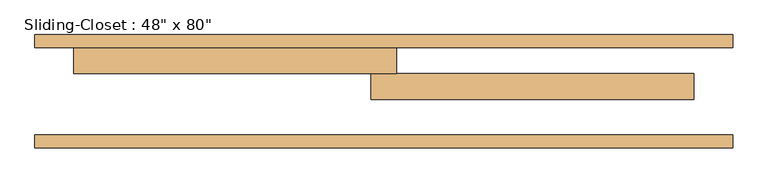
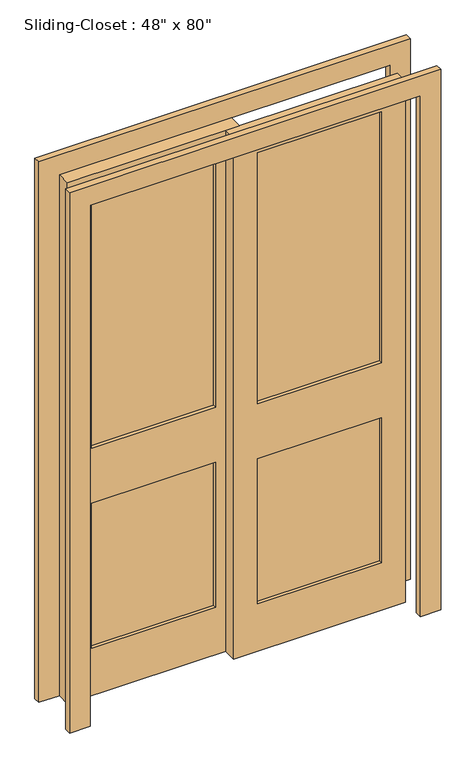
"""IFC4 building model written with IfcOpenShell, lengths in millimetres: door geometry."""

from ifc_helpers import new_model, si_unit, frame, origin, place, context, project, spatial, polyline, outline, extrude, source, transform, mapped, element, save


def door_89925928(model_context):
    return source(origin(), model_context, "Body", "SweptSolid", [
        extrude(outline(polyline([(-63.5, 174.625), (-520.7, 174.625), (-520.7, 200.025), (-63.5, 200.025), (-63.5, 174.625)])), frame((0.0, 0.0, 965.2), z_axis=(0.0, 0.0, 1.0), x_axis=(1.0, 0.0, 0.0)), (0.0, 0.0, 1.0), 977.9),
        extrude(outline(polyline([(-63.5, 174.625), (-520.7, 174.625), (-520.7, 200.025), (-63.5, 200.025), (-63.5, 174.625)])), frame((0.0, 0.0, 184.15), z_axis=(0.0, 0.0, 1.0), x_axis=(1.0, 0.0, 0.0)), (0.0, 0.0, 1.0), 565.15),
        extrude(outline(polyline([(63.5, 149.225), (520.7, 149.225), (520.7, 123.825), (63.5, 123.825), (63.5, 149.225)])), frame((0.0, 0.0, 965.2), z_axis=(0.0, 0.0, 1.0), x_axis=(1.0, 0.0, 0.0)), (0.0, 0.0, 1.0), 977.9),
        extrude(outline(polyline([(63.5, 149.225), (520.7, 149.225), (520.7, 123.825), (63.5, 123.825), (63.5, 149.225)])), frame((0.0, 0.0, 184.15), z_axis=(0.0, 0.0, 1.0), x_axis=(1.0, 0.0, 0.0)), (0.0, 0.0, 1.0), 565.15),
        extrude(outline(polyline([(2032.0, 25.4), (2032.0, -609.6), (0.0, -609.6), (0.0, 25.4), (2032.0, 25.4)]), holes=[polyline([(184.15, -520.7), (749.3, -520.7), (749.3, -63.5), (184.15, -63.5), (184.15, -520.7)]), polyline([(965.2, -520.7), (1943.1, -520.7), (1943.1, -63.5), (965.2, -63.5), (965.2, -520.7)])]), frame((0.0, 161.925, 0.0), z_axis=(0.0, 1.0, 0.0), x_axis=(0.0, 0.0, 1.0)), (0.0, 0.0, 1.0), 50.8),
        extrude(outline(polyline([(0.0, -685.8), (0.0, -609.6), (2032.0, -609.6), (2032.0, 609.6), (0.0, 609.6), (0.0, 685.8), (2108.2, 685.8), (2108.2, -685.8), (0.0, -685.8)])), frame((0.0, 15.875, 0.0), z_axis=(0.0, 1.0, 0.0), x_axis=(0.0, 0.0, 1.0)), (0.0, 0.0, 1.0), 25.4),
        extrude(outline(polyline([(0.0, 685.8), (2108.2, 685.8), (2108.2, -685.8), (0.0, -685.8), (0.0, -609.6), (2032.0, -609.6), (2032.0, 609.6), (0.0, 609.6), (0.0, 685.8)])), frame((0.0, 212.725, 0.0), z_axis=(0.0, 1.0, 0.0), x_axis=(0.0, 0.0, 1.0)), (0.0, 0.0, 1.0), 25.4),
        extrude(outline(polyline([(2032.0, -25.4), (0.0, -25.4), (0.0, 609.6), (2032.0, 609.6), (2032.0, -25.4)]), holes=[polyline([(965.2, 520.7), (965.2, 63.5), (1943.1, 63.5), (1943.1, 520.7), (965.2, 520.7)]), polyline([(184.15, 520.7), (184.15, 63.5), (749.3, 63.5), (749.3, 520.7), (184.15, 520.7)])]), frame((0.0, 111.125, 0.0), z_axis=(0.0, 1.0, 0.0), x_axis=(0.0, 0.0, 1.0)), (0.0, 0.0, 1.0), 50.8),
    ])


if __name__ == "__main__":
    model = new_model("IFC4")
    model_context = context("Model", 3, world=origin())
    ifc_project = project(units=[si_unit("LENGTHUNIT", "METRE", prefix="MILLI")], contexts=[model_context])
    site = spatial("IfcSite", under=ifc_project)
    building = spatial("IfcBuilding", under=site)
    placement = place(None, origin())
    door_shape = door_89925928(model_context)
    element("IfcDoor", 1, ObjectType="Sliding-Closet : 48\" x 80\"", at=placement, inside=building, context=model_context, shape_type="MappedRepresentation", body=[
        mapped(door_shape, transform((0.0, 0.0, 0.0), x_axis=(1.0, 0.0, 0.0), y_axis=(0.0, 1.0, 0.0), z_axis=(0.0, 0.0, 1.0))),
    ])
    save(model, "model.ifc")

# Revit data of these elements
# Type "Sliding-Closet : 48\" x 80\""
#   Type Mark = "54"
#   Assembly Code = "C1020"
#   Thickness = 0' - 2"
#   Height = 6' - 8"
#   Trim Projection Ext = 0' - 1"
#   Trim Projection Int = 0' - 1"
#   Trim Width = 0' - 3"
#   Width = 4' - 0"
#   Define Thermal Properties by = 0
#   Function = 0
#   Door Material = Door - Panel
#   Frame Material = Door - Frame
#   Wall Closure = (empty or 0)
# Element 1 (IfcDoor, "Sliding-Closet : 48\" x 80\"")
#   Materials on its faces: "Door - Panel", "Door - Frame"
# Materials
#   "Door - Panel": class "Wood", colour RGB 227 170 128, transparency 0, Cost = 0
#   "Door - Frame": class "Miscellaneous", colour RGB 153 76 43, transparency 0, Cost = 0
